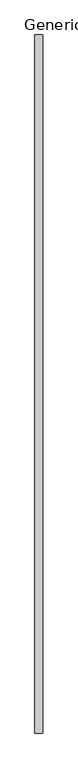
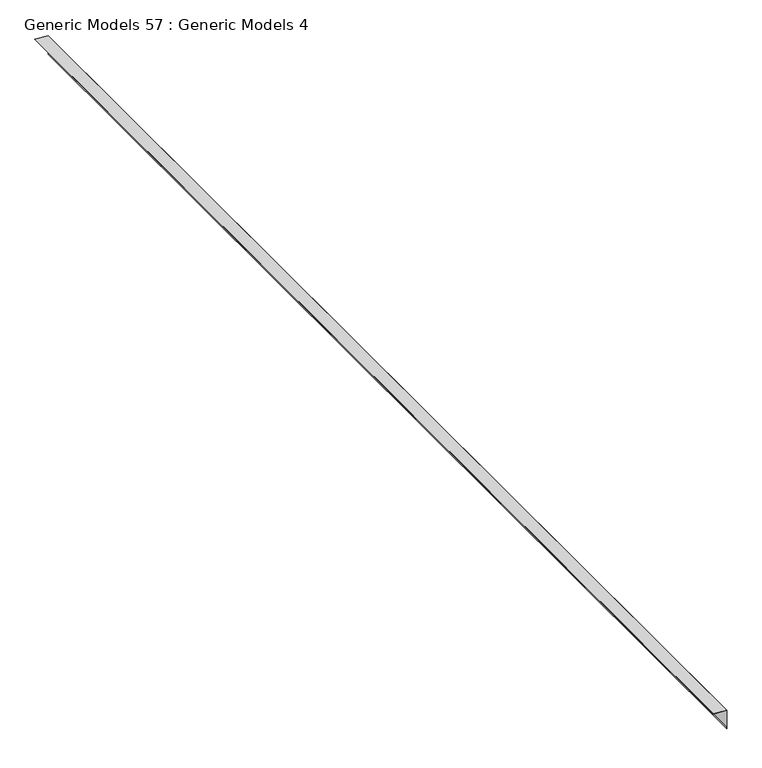
"""IFC4 building model written with IfcOpenShell, lengths in millimetres: proxy geometry, Generic Models 57 : Generic Models 4."""

from ifc_helpers import new_model, si_unit, frame, origin, place, context, project, spatial, polyline, outline, extrude, source, transform, mapped, element, save


def generic_models_57_generic_models_4_05ee7690(model_context):
    return source(origin(), model_context, "Body", "SweptSolid", [
        extrude(outline(polyline([(126712.1725001, -9253.0996905), (126693.1385401, -9253.0996905), (126693.1385401, -9252.3059405), (126712.3124596, -9252.3059405), (126719.4444002, -9254.9017545), (126926.0813226, -9254.9017545), (126932.6803171, -9413.2776217), (126931.8872552, -9413.310666), (126925.3199568, -9255.6955045), (126719.3044406, -9255.6955045), (126712.1725001, -9253.0996905)])), frame((0.0, -6864.9230338, 0.0), z_axis=(0.0, 1.0, 0.0), x_axis=(0.0, 0.0, 1.0)), (0.0, 0.0, 1.0), 13919.2),
    ])


if __name__ == "__main__":
    model = new_model("IFC4")
    model_context = context("Model", 3, world=origin())
    ifc_project = project(units=[si_unit("LENGTHUNIT", "METRE", prefix="MILLI")], contexts=[model_context])
    site = spatial("IfcSite", under=ifc_project)
    building = spatial("IfcBuilding", under=site)
    placement = place(None, origin())
    generic_models_57_generic_models_4_shape = generic_models_57_generic_models_4_05ee7690(model_context)
    element("IfcBuildingElementProxy", 1, Name="Generic Models 57 : Generic Models 4", ObjectType="Generic Models 57 : Generic Models 4", at=placement, inside=building, context=model_context, shape_type="MappedRepresentation", body=[
        mapped(generic_models_57_generic_models_4_shape, transform((0.0, 0.0, 0.0), x_axis=(1.0, 0.0, 0.0), y_axis=(0.0, 1.0, 0.0), z_axis=(0.0, 0.0, 1.0))),
    ])
    save(model, "model.ifc")

# Revit data of these elements
# Element 1 (IfcBuildingElementProxy, "Generic Models 57 : Generic Models 4")
#   Materials on its faces: "_(2) LAYERS NO. 30 ASTM D226 ASPHALT SATURATED ORGANIC FELT"
# Materials
#   "_(2) LAYERS NO. 30 ASTM D226 ASPHALT SATURATED ORGANIC FELT": class "Generic", colour RGB 67 154 161, transparency 0, Cost = 0
